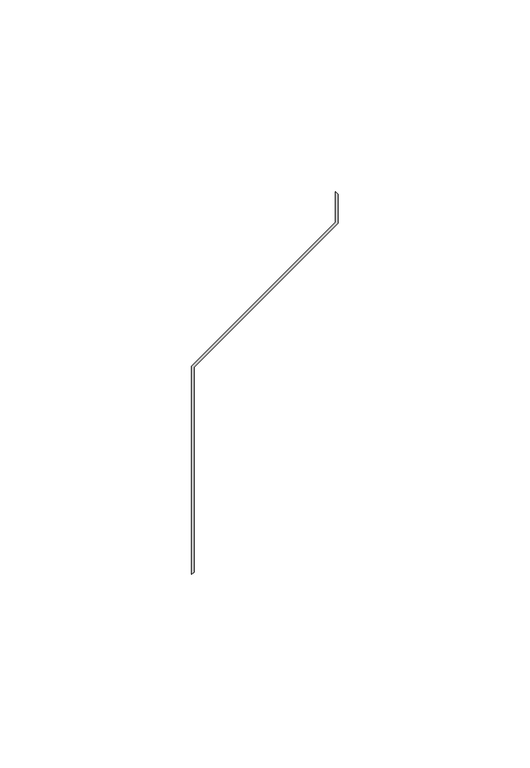
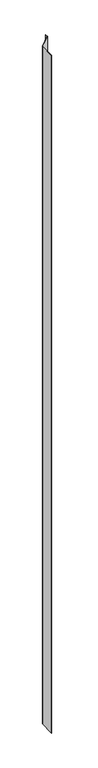
"""IFC4 building model written with IfcOpenShell, lengths in millimetres: proxy geometry, MBCI 7.2-V Panel4 : MBCI 7.2-V Panel-1."""

from ifc_helpers import new_model, si_unit, frame, origin, place, context, project, spatial, polyline, outline, extrude, source, transform, mapped, element, save


def generic_models_61abd2db(model_context):
    return source(origin(), model_context, "Body", "SweptSolid", [
        extrude(outline(polyline([(587328.4903864, -536352.8639068), (587328.4903864, -536406.3026716), (587327.8950739, -536406.8979841), (587327.8950739, -536352.6173202), (587365.3854739, -536315.1269202), (587365.3854739, -536307.2537841), (587365.9807864, -536307.8490966), (587365.9807864, -536315.3735068), (587328.4903864, -536352.8639068)])), frame((0.0, 0.0, 12.7), z_axis=(0.0, 0.0, 1.0), x_axis=(1.0, 0.0, 0.0)), (0.0, 0.0, 1.0), 2425.7),
    ])


if __name__ == "__main__":
    model = new_model("IFC4")
    model_context = context("Model", 3, world=origin())
    ifc_project = project(units=[si_unit("LENGTHUNIT", "METRE", prefix="MILLI")], contexts=[model_context])
    site = spatial("IfcSite", under=ifc_project)
    building = spatial("IfcBuilding", under=site)
    placement = place(None, origin())
    generic_models_shape = generic_models_61abd2db(model_context)
    element("IfcBuildingElementProxy", 1, Name="MBCI 7.2-V Panel4 : MBCI 7.2-V Panel-1", ObjectType="MBCI 7.2-V Panel4 : MBCI 7.2-V Panel-1", at=placement, inside=building, context=model_context, shape_type="MappedRepresentation", body=[
        mapped(generic_models_shape, transform((0.0, 0.0, 0.0), x_axis=(1.0, 0.0, 0.0), y_axis=(0.0, 1.0, 0.0), z_axis=(0.0, 0.0, 1.0))),
    ])
    save(model, "model.ifc")

# Revit data of these elements
# Element 1 (IfcBuildingElementProxy, "MBCI 7.2-V Panel4 : MBCI 7.2-V Panel-1")
#   Materials on its faces: "MTL PANEL"
# Materials
#   "MTL PANEL": class "Generic", colour RGB 239 242 240, transparency 0, Cost = 0
